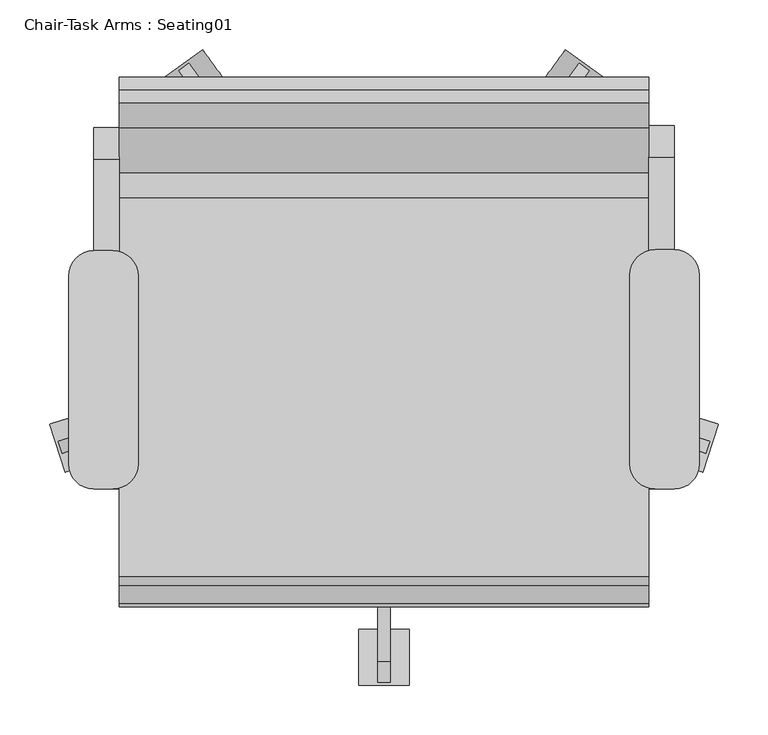
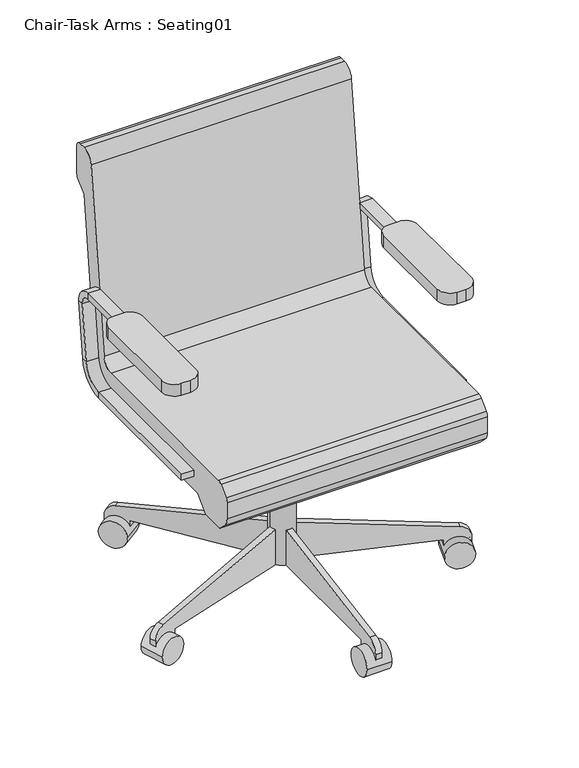
"""IFC4 building model written with IfcOpenShell, lengths in millimetres: furniture geometry, Chair-Task Arms : Seating01."""

from ifc_helpers import new_model, si_unit, point, frame, frame_2d, origin, place, context, project, spatial, polyline, circle_curve, trimmed, segment, composite_curve, outline, extrude, source, transform, mapped, element, save
from ifc_brep_helpers import plane_surface, cylinder_surface, revolved_surface, advanced_brep


def chair_task_arms_seating01_8395c10b(model_context):
    return source(origin(), model_context, "Body", "SolidModel", [
        extrude(outline(composite_curve([segment(trimmed(circle_curve(frame_2d((433.0908197, 48.8028048)), 25.4), [point((433.0908197, 74.2028048))], [point((458.4908197, 48.8028048))], False, "CARTESIAN"), True, "CONTINUOUS"), segment(polyline([(458.4908197, 48.8028048), (458.4908197, -141.6319091)]), True, "CONTINUOUS"), segment(trimmed(circle_curve(frame_2d((433.0908197, -141.6319091)), 25.4), [point((458.4908197, -141.6319091))], [point((433.0908197, -167.0319091))], False, "CARTESIAN"), True, "CONTINUOUS"), segment(polyline([(433.0908197, -167.0319091), (414.0408197, -167.0319091)]), True, "CONTINUOUS"), segment(trimmed(circle_curve(frame_2d((414.0408197, -141.6319091)), 25.4), [point((414.0408197, -167.0319091))], [point((388.6408197, -141.6319091))], False, "CARTESIAN"), True, "CONTINUOUS"), segment(polyline([(388.6408197, -141.6319091), (388.6408197, 48.8028048)]), True, "CONTINUOUS"), segment(trimmed(circle_curve(frame_2d((414.0408197, 48.8028048)), 25.4), [point((388.6408197, 48.8028048))], [point((414.0408197, 74.2028048))], False, "CARTESIAN"), True, "CONTINUOUS"), segment(polyline([(414.0408197, 74.2028048), (433.0908197, 74.2028048)]), True, "CONTINUOUS")], self_intersect=False)), frame((0.0, 0.0, 596.9), z_axis=(0.0, 0.0, 1.0), x_axis=(1.0, 0.0, 0.0)), (0.0, 0.0, 1.0), 25.4),
        extrude(outline(composite_curve([segment(trimmed(circle_curve(frame_2d((-132.0591803, 47.7575984)), 25.4), [point((-132.0591803, 73.1575984))], [point((-106.6591803, 47.7575984))], False, "CARTESIAN"), True, "CONTINUOUS"), segment(polyline([(-106.6591803, 47.7575984), (-106.6591803, -141.6319091)]), True, "CONTINUOUS"), segment(trimmed(circle_curve(frame_2d((-132.0591803, -141.6319091)), 25.4), [point((-106.6591803, -141.6319091))], [point((-132.0591803, -167.0319091))], False, "CARTESIAN"), True, "CONTINUOUS"), segment(polyline([(-132.0591803, -167.0319091), (-151.1091803, -167.0319091)]), True, "CONTINUOUS"), segment(trimmed(circle_curve(frame_2d((-151.1091803, -141.6319091)), 25.4), [point((-151.1091803, -167.0319091))], [point((-176.5091803, -141.6319091))], False, "CARTESIAN"), True, "CONTINUOUS"), segment(polyline([(-176.5091803, -141.6319091), (-176.5091803, 47.7575984)]), True, "CONTINUOUS"), segment(trimmed(circle_curve(frame_2d((-151.1091803, 47.7575984)), 25.4), [point((-176.5091803, 47.7575984))], [point((-151.1091803, 73.1575984))], False, "CARTESIAN"), True, "CONTINUOUS"), segment(polyline([(-151.1091803, 73.1575984), (-132.0591803, 73.1575984)]), True, "CONTINUOUS")], self_intersect=False)), frame((0.0, 0.0, 596.9), z_axis=(0.0, 0.0, 1.0), x_axis=(1.0, 0.0, 0.0)), (0.0, 0.0, 1.0), 25.4),
        advanced_brep(
        [(-151.1091803, -167.0319091, 412.75), (-125.7091803, -167.0319091, 412.75), (-125.7091803, -167.0319091, 425.45), (-151.1091803, -167.0319091, 425.45), (-151.1091803, 126.2388651, 425.45), (-151.1091803, 126.2388651, 412.75), (-125.7091803, 126.2388651, 425.45), (-125.7091803, 126.2388651, 412.75), (-151.1091803, 170.3844094, 464.7064065), (-151.1091803, 182.9974221, 463.2225227), (-125.7091803, 170.3844094, 464.7064065), (-125.7091803, 182.9974221, 463.2225227), (-151.1091803, 184.1806174, 581.9741742), (-151.1091803, 196.7936301, 580.4902904), (-125.7091803, 184.1806174, 581.9741742), (-125.7091803, 196.7936301, 580.4902904), (-151.1091803, 165.2610984, 603.25), (-151.1091803, 165.2610984, 615.95), (-125.7091803, 165.2610984, 603.25), (-125.7091803, 165.2610984, 615.95), (-151.1091803, -18.9459016, 615.95), (-151.1091803, -18.9459016, 603.25), (-125.7091803, -18.9459016, 603.25), (-125.7091803, -18.9459016, 615.95)],
        [
            (0, 1),
            (1, 2),
            (2, 3),
            (3, 0),
            (3, 4),
            (4, 5),
            (5, 0),
            (2, 6),
            (6, 4),
            (1, 7),
            (7, 6),
            (5, 7),
            (8, 9),
            (9, 5, circle_curve(frame((-151.1091803, 126.2388651, 469.9), z_axis=(-1.0, 0.0, 0.0), x_axis=(0.0, 0.0, -1.0)), 57.15)),
            (4, 8, circle_curve(frame((-151.1091803, 126.2388651, 469.9), z_axis=(1.0, 0.0, 0.0), x_axis=(0.0, 0.0, -1.0)), 44.45)),
            (10, 8),
            (6, 10, circle_curve(frame((-125.7091803, 126.2388651, 469.9), z_axis=(1.0, 0.0, 0.0), x_axis=(0.0, 0.0, -1.0)), 44.45)),
            (11, 10),
            (7, 11, circle_curve(frame((-125.7091803, 126.2388651, 469.9), z_axis=(1.0, 0.0, 0.0), x_axis=(0.0, 0.0, -1.0)), 57.15)),
            (9, 11),
            (8, 12),
            (12, 13),
            (13, 9),
            (10, 14),
            (14, 12),
            (11, 15),
            (15, 14),
            (13, 15),
            (16, 17),
            (17, 13, circle_curve(frame((-151.1091803, 165.2610984, 584.2), z_axis=(-1.0, 0.0, 0.0), x_axis=(0.0, 0.9931506043228768, -0.11684124756739202)), 31.75)),
            (12, 16, circle_curve(frame((-151.1091803, 165.2610984, 584.2), z_axis=(1.0, 0.0, 0.0), x_axis=(0.0, 0.9931506043228768, -0.11684124756739202)), 19.05)),
            (18, 16),
            (14, 18, circle_curve(frame((-125.7091803, 165.2610984, 584.2), z_axis=(1.0, 0.0, 0.0), x_axis=(0.0, 0.9931506043228768, -0.11684124756739202)), 19.05)),
            (19, 18),
            (15, 19, circle_curve(frame((-125.7091803, 165.2610984, 584.2), z_axis=(1.0, 0.0, 0.0), x_axis=(0.0, 0.9931506043228768, -0.11684124756739202)), 31.75)),
            (17, 19),
            (20, 21),
            (21, 22),
            (22, 23),
            (23, 20),
            (16, 21),
            (20, 17),
            (18, 22),
            (19, 23),
        ],
        [
            plane_surface(frame((-152.608212, -167.0319091, 419.1), z_axis=(0.0, -1.0, 0.0), x_axis=(0.0, 0.0, -1.0))),
            plane_surface(frame((-151.1091803, -167.0319091, 412.75), z_axis=(-1.0, 0.0, 0.0), x_axis=(0.0, 1.0, 0.0))),
            plane_surface(frame((-151.1091803, -167.0319091, 425.45), z_axis=(0.0, 0.0, 1.0), x_axis=(0.0, 1.0, 0.0))),
            plane_surface(frame((-125.7091803, -167.0319091, 425.45), z_axis=(1.0, 0.0, 0.0), x_axis=(0.0, 1.0, 0.0))),
            plane_surface(frame((-125.7091803, -167.0319091, 412.75), z_axis=(0.0, 0.0, -1.0), x_axis=(0.0, 1.0, 0.0))),
            plane_surface(frame((-151.1091803, 126.2388651, 469.9), z_axis=(-1.0, 0.0, 0.0), x_axis=(0.0, 0.0, -1.0))),
            revolved_surface(polyline([(-151.1091803, 126.2388651, 425.45), (-125.7091803, 126.2388651, 425.45)]), (-138.4091803, 126.2388651, 469.9), (-1.0, 0.0, 0.0)),
            plane_surface(frame((-125.7091803, 126.2388651, 469.9), z_axis=(1.0, 0.0, 0.0), x_axis=(0.0, 0.0, -1.0))),
            cylinder_surface(frame((-138.4091803, 126.2388651, 469.9), z_axis=(-1.0, 0.0, 0.0), x_axis=(0.0, 0.0, -1.0)), 57.15),
            plane_surface(frame((-151.1091803, 182.9974221, 463.2225227), z_axis=(-1.0, 0.0, 0.0), x_axis=(0.0, 0.1168412475673856, 0.9931506043228776))),
            plane_surface(frame((-151.1091803, 170.3844094, 464.7064065), z_axis=(0.0, -0.9931506043228776, 0.1168412475673856), x_axis=(0.0, 0.1168412475673856, 0.9931506043228776))),
            plane_surface(frame((-125.7091803, 170.3844094, 464.7064065), z_axis=(1.0, 0.0, 0.0), x_axis=(0.0, 0.1168412475673856, 0.9931506043228776))),
            plane_surface(frame((-125.7091803, 182.9974221, 463.2225227), z_axis=(0.0, 0.9931506043228776, -0.1168412475673856), x_axis=(0.0, 0.1168412475673856, 0.9931506043228776))),
            plane_surface(frame((-151.1091803, 165.2610984, 584.2), z_axis=(-1.0, 0.0, 0.0), x_axis=(0.0, 0.9931506043228768, -0.11684124756739202))),
            revolved_surface(polyline([(-151.1091803, 184.1806174123508, 581.9741742338413), (-125.7091803, 184.1806174123508, 581.9741742338413)]), (-138.4091803, 165.2610984, 584.2), (-1.0, 0.0, 0.0)),
            plane_surface(frame((-125.7091803, 165.2610984, 584.2), z_axis=(1.0, 0.0, 0.0), x_axis=(0.0, 0.9931506043228768, -0.11684124756739202))),
            cylinder_surface(frame((-138.4091803, 165.2610984, 584.2), z_axis=(-1.0, 0.0, 0.0), x_axis=(0.0, 0.9931506043228768, -0.11684124756739202)), 31.75),
            plane_surface(frame((-152.608212, -18.9459016, 609.6), z_axis=(0.0, -1.0, 0.0), x_axis=(0.0, 0.0, 1.0))),
            plane_surface(frame((-151.1091803, 165.2610984, 615.95), z_axis=(-1.0, 0.0, 0.0), x_axis=(0.0, -1.0, 0.0))),
            plane_surface(frame((-151.1091803, 165.2610984, 603.25), z_axis=(0.0, 0.0, -1.0), x_axis=(0.0, -1.0, 0.0))),
            plane_surface(frame((-125.7091803, 165.2610984, 603.25), z_axis=(1.0, 0.0, 0.0), x_axis=(0.0, -1.0, 0.0))),
            plane_surface(frame((-125.7091803, 165.2610984, 615.95), z_axis=(0.0, 0.0, 1.0), x_axis=(0.0, -1.0, 0.0))),
        ],
        [
            (0, [[1, 2, 3, 4]]),
            (1, [[5, 6, 7, -4]]),
            (2, [[8, 9, -5, -3]]),
            (3, [[10, 11, -8, -2]]),
            (4, [[-7, 12, -10, -1]]),
            (5, [[13, 14, -6, 15]]),
            (6, [[16, -15, -9, 17]]),
            (7, [[18, -17, -11, 19]]),
            (8, [[20, -19, -12, -14]]),
            (9, [[21, 22, 23, -13]]),
            (10, [[24, 25, -21, -16]]),
            (11, [[26, 27, -24, -18]]),
            (12, [[-23, 28, -26, -20]]),
            (13, [[29, 30, -22, 31]]),
            (14, [[32, -31, -25, 33]]),
            (15, [[34, -33, -27, 35]]),
            (16, [[36, -35, -28, -30]]),
            (17, [[37, 38, 39, 40]]),
            (18, [[41, -37, 42, -29]]),
            (19, [[43, -38, -41, -32]]),
            (20, [[44, -39, -43, -34]]),
            (21, [[-42, -40, -44, -36]]),
        ],
    ),
        advanced_brep(
        [(433.0908197, -167.0319091, 425.45), (407.6908197, -167.0319091, 425.45), (407.6908197, -167.0319091, 412.75), (433.0908197, -167.0319091, 412.75), (433.0908197, 128.329278, 412.75), (433.0908197, 128.329278, 425.45), (407.6908197, 128.329278, 412.75), (407.6908197, 128.329278, 425.45), (433.0908197, 185.0878351, 463.2225227), (433.0908197, 172.4748224, 464.7064065), (407.6908197, 185.0878351, 463.2225227), (407.6908197, 172.4748224, 464.7064065), (433.0908197, 198.884043, 580.4902904), (433.0908197, 186.2710303, 581.9741742), (407.6908197, 198.884043, 580.4902904), (407.6908197, 186.2710303, 581.9741742), (433.0908197, 167.3515113, 615.95), (433.0908197, 167.3515113, 603.25), (407.6908197, 167.3515113, 615.95), (407.6908197, 167.3515113, 603.25), (433.0908197, -18.9459016, 603.25), (433.0908197, -18.9459016, 615.95), (407.6908197, -18.9459016, 615.95), (407.6908197, -18.9459016, 603.25)],
        [
            (0, 1),
            (1, 2),
            (2, 3),
            (3, 0),
            (3, 4),
            (4, 5),
            (5, 0),
            (2, 6),
            (6, 4),
            (1, 7),
            (7, 6),
            (5, 7),
            (8, 9),
            (9, 5, circle_curve(frame((433.0908197, 128.329278, 469.9), z_axis=(-1.0, 0.0, 0.0), x_axis=(0.0, 0.0, -1.0)), 44.45)),
            (4, 8, circle_curve(frame((433.0908197, 128.329278, 469.9), z_axis=(1.0, 0.0, 0.0), x_axis=(0.0, 0.0, -1.0)), 57.15)),
            (10, 8),
            (6, 10, circle_curve(frame((407.6908197, 128.329278, 469.9), z_axis=(1.0, 0.0, 0.0), x_axis=(0.0, 0.0, -1.0)), 57.15)),
            (11, 10),
            (7, 11, circle_curve(frame((407.6908197, 128.329278, 469.9), z_axis=(1.0, 0.0, 0.0), x_axis=(0.0, 0.0, -1.0)), 44.45)),
            (9, 11),
            (8, 12),
            (12, 13),
            (13, 9),
            (10, 14),
            (14, 12),
            (11, 15),
            (15, 14),
            (13, 15),
            (16, 17),
            (17, 13, circle_curve(frame((433.0908197, 167.3515113, 584.2), z_axis=(-1.0, 0.0, 0.0), x_axis=(0.0, 0.9931506043228767, -0.1168412475673929)), 19.05)),
            (12, 16, circle_curve(frame((433.0908197, 167.3515113, 584.2), z_axis=(1.0, 0.0, 0.0), x_axis=(0.0, 0.9931506043228767, -0.1168412475673929)), 31.75)),
            (18, 16),
            (14, 18, circle_curve(frame((407.6908197, 167.3515113, 584.2), z_axis=(1.0, 0.0, 0.0), x_axis=(0.0, 0.9931506043228767, -0.1168412475673929)), 31.75)),
            (19, 18),
            (15, 19, circle_curve(frame((407.6908197, 167.3515113, 584.2), z_axis=(1.0, 0.0, 0.0), x_axis=(0.0, 0.9931506043228767, -0.1168412475673929)), 19.05)),
            (17, 19),
            (20, 21),
            (21, 22),
            (22, 23),
            (23, 20),
            (16, 21),
            (20, 17),
            (18, 22),
            (19, 23),
        ],
        [
            plane_surface(frame((406.191788, -167.0319091, 419.1), z_axis=(0.0, -1.0, 0.0), x_axis=(0.0, 0.0, -1.0))),
            plane_surface(frame((433.0908197, -167.0319091, 425.45), z_axis=(1.0, 0.0, 0.0), x_axis=(0.0, 1.0, 0.0))),
            plane_surface(frame((433.0908197, -167.0319091, 412.75), z_axis=(0.0, 0.0, -1.0), x_axis=(0.0, 1.0, 0.0))),
            plane_surface(frame((407.6908197, -167.0319091, 412.75), z_axis=(-1.0, 0.0, 0.0), x_axis=(0.0, 1.0, 0.0))),
            plane_surface(frame((407.6908197, -167.0319091, 425.45), z_axis=(0.0, 0.0, 1.0), x_axis=(0.0, 1.0, 0.0))),
            plane_surface(frame((433.0908197, 128.329278, 469.9), z_axis=(1.0, 0.0, 0.0), x_axis=(0.0, 0.0, -1.0))),
            cylinder_surface(frame((420.3908197, 128.329278, 469.9), z_axis=(-1.0, 0.0, 0.0), x_axis=(0.0, 0.0, -1.0)), 57.15),
            plane_surface(frame((407.6908197, 128.329278, 469.9), z_axis=(-1.0, 0.0, 0.0), x_axis=(0.0, 0.0, -1.0))),
            revolved_surface(polyline([(407.6908197, 128.329278, 425.45), (433.0908197, 128.329278, 425.45)]), (420.3908197, 128.329278, 469.9), (-1.0, 0.0, 0.0)),
            plane_surface(frame((433.0908197, 172.4748224, 464.7064065), z_axis=(1.0, 0.0, 0.0), x_axis=(0.0, 0.11684124756738626, 0.9931506043228775))),
            plane_surface(frame((433.0908197, 185.0878351, 463.2225227), z_axis=(0.0, 0.9931506043228775, -0.11684124756738619), x_axis=(0.0, 0.11684124756738619, 0.9931506043228775))),
            plane_surface(frame((407.6908197, 185.0878351, 463.2225227), z_axis=(-1.0, 0.0, 0.0), x_axis=(0.0, 0.11684124756738619, 0.9931506043228775))),
            plane_surface(frame((407.6908197, 172.4748224, 464.7064065), z_axis=(0.0, -0.9931506043228775, 0.11684124756738626), x_axis=(0.0, 0.11684124756738626, 0.9931506043228775))),
            plane_surface(frame((433.0908197, 167.3515113, 584.2), z_axis=(1.0, 0.0, 0.0), x_axis=(0.0, 0.9931506043228767, -0.1168412475673929))),
            cylinder_surface(frame((420.3908197, 167.3515113, 584.2), z_axis=(-1.0, 0.0, 0.0), x_axis=(0.0, 0.9931506043228767, -0.1168412475673929)), 31.75),
            plane_surface(frame((407.6908197, 167.3515113, 584.2), z_axis=(-1.0, 0.0, 0.0), x_axis=(0.0, 0.9931506043228767, -0.1168412475673929))),
            revolved_surface(polyline([(407.6908197, 186.2710303123508, 581.9741742338412), (433.0908197, 186.2710303123508, 581.9741742338412)]), (420.3908197, 167.3515113, 584.2), (-1.0, 0.0, 0.0)),
            plane_surface(frame((406.191788, -18.9459016, 609.6), z_axis=(0.0, -1.0, 0.0), x_axis=(0.0, 0.0, 1.0))),
            plane_surface(frame((433.0908197, 167.3515113, 603.25), z_axis=(1.0, 0.0, 0.0), x_axis=(0.0, -1.0, 0.0))),
            plane_surface(frame((433.0908197, 167.3515113, 615.95), z_axis=(0.0, 0.0, 1.0), x_axis=(0.0, -1.0, 0.0))),
            plane_surface(frame((407.6908197, 167.3515113, 615.95), z_axis=(-1.0, 0.0, 0.0), x_axis=(0.0, -1.0, 0.0))),
            plane_surface(frame((407.6908197, 167.3515113, 603.25), z_axis=(0.0, 0.0, -1.0), x_axis=(0.0, -1.0, 0.0))),
        ],
        [
            (0, [[1, 2, 3, 4]]),
            (1, [[5, 6, 7, -4]]),
            (2, [[8, 9, -5, -3]]),
            (3, [[10, 11, -8, -2]]),
            (4, [[-7, 12, -10, -1]]),
            (5, [[13, 14, -6, 15]]),
            (6, [[16, -15, -9, 17]]),
            (7, [[18, -17, -11, 19]]),
            (8, [[20, -19, -12, -14]]),
            (9, [[21, 22, 23, -13]]),
            (10, [[24, 25, -21, -16]]),
            (11, [[26, 27, -24, -18]]),
            (12, [[-23, 28, -26, -20]]),
            (13, [[29, 30, -22, 31]]),
            (14, [[32, -31, -25, 33]]),
            (15, [[34, -33, -27, 35]]),
            (16, [[36, -35, -28, -30]]),
            (17, [[37, 38, 39, 40]]),
            (18, [[41, -37, 42, -29]]),
            (19, [[43, -38, -41, -32]]),
            (20, [[44, -39, -43, -34]]),
            (21, [[-42, -40, -44, -36]]),
        ],
    ),
        extrude(outline(composite_curve([segment(trimmed(circle_curve(frame_2d((140.9908197, -18.9459016)), 25.4), [point((115.5908197, -18.9459016))], [point((166.3908197, -18.9459016))], False, "CARTESIAN"), True, "CONTINUOUS"), segment(trimmed(circle_curve(frame_2d((140.9908197, -18.9459016)), 25.4), [point((166.3908197, -18.9459016))], [point((115.5908197, -18.9459016))], False, "CARTESIAN"), True, "CONTINUOUS")], self_intersect=False)), frame((0.0, 0.0, 53.5835944), z_axis=(0.0, 0.0, 1.0), x_axis=(1.0, 0.0, 0.0)), (0.0, 0.0, 1.0), 330.5914056),
        extrude(outline(composite_curve([segment(trimmed(circle_curve(frame_2d((0.0, 28.2002728)), 28.2002727), [point((0.0, 56.4005455))], [point((0.0, 0.0))], False, "CARTESIAN"), True, "CONTINUOUS"), segment(trimmed(circle_curve(frame_2d((0.0, 28.2002728)), 28.2002727), [point((0.0, 0.0))], [point((0.0, 56.4005455))], False, "CARTESIAN"), True, "CONTINUOUS")], self_intersect=False)), frame((461.9222851, -149.9299964, 28.1835944), z_axis=(0.3090169943749423, 0.9510565162951553, 0.0), x_axis=(0.0, 0.0, -1.0)), (0.0, 0.0, 1.0), 50.8),
        extrude(outline(composite_curve([segment(polyline([(25.4, 0.0), (0.0, 0.0), (0.0, 50.8), (24.303053, 50.8)]), True, "CONTINUOUS"), segment(trimmed(circle_curve(frame_2d((24.303053, 25.4)), 25.4), [point((24.303053, 50.8))], [point((49.3171699, 29.8106636))], False, "CARTESIAN"), True, "CONTINUOUS"), segment(polyline([(49.3171699, 29.8106636), (101.6, -266.7), (101.6, -292.1), (25.4, -292.1), (25.4, 0.0)]), True, "CONTINUOUS")], self_intersect=False)), frame((416.8321702, -115.2489746, 28.1835944), z_axis=(0.3090169943749423, 0.9510565162951553, 0.0), x_axis=(0.0, 0.0, 1.0)), (0.0, 0.0, 1.0), 12.7),
        extrude(outline(composite_curve([segment(trimmed(circle_curve(frame_2d((0.0, 28.2002726)), 28.2002727), [point((0.0, 56.4005454))], [point((0.0, 0.0))], False, "CARTESIAN"), True, "CONTINUOUS"), segment(trimmed(circle_curve(frame_2d((0.0, 28.2002726)), 28.2002727), [point((0.0, 0.0))], [point((0.0, 56.4005454))], False, "CARTESIAN"), True, "CONTINUOUS")], self_intersect=False)), frame((364.7373733, 245.8017485, 28.1835944), z_axis=(-0.8090169943749499, 0.5877852522924699, 0.0), x_axis=(0.0, 0.0, -1.0)), (0.0, 0.0, 1.0), 50.8),
        extrude(outline(composite_curve([segment(polyline([(25.4, 0.0), (0.0, 0.0), (0.0, 50.8), (24.303053, 50.8)]), True, "CONTINUOUS"), segment(trimmed(circle_curve(frame_2d((24.303053, 25.3999999)), 25.4), [point((24.303053, 50.8))], [point((49.3171699, 29.8106637))], False, "CARTESIAN"), True, "CONTINUOUS"), segment(polyline([(49.3171699, 29.8106637), (101.6, -266.7), (101.6, -292.1), (25.4, -292.1), (25.4, 0.0)]), True, "CONTINUOUS")], self_intersect=False)), frame((317.8201498, 213.6355261, 28.1835944), z_axis=(-0.8090169943749499, 0.5877852522924699, 0.0), x_axis=(0.0, 0.0, 1.0)), (0.0, 0.0, 1.0), 12.7),
        extrude(outline(composite_curve([segment(trimmed(circle_curve(frame_2d((0.0, 28.2002726)), 28.2002727), [point((0.0, 56.4005454))], [point((0.0, 0.0))], False, "CARTESIAN"), True, "CONTINUOUS"), segment(trimmed(circle_curve(frame_2d((0.0, 28.2002726)), 28.2002727), [point((0.0, 0.0))], [point((0.0, 56.4005454))], False, "CARTESIAN"), True, "CONTINUOUS")], self_intersect=False)), frame((-82.755734, 245.8017485, 28.1835944), z_axis=(0.8090169943749458, 0.5877852522924754, 0.0), x_axis=(0.0, 0.0, 1.0)), (0.0, 0.0, 1.0), 50.8),
        extrude(outline(composite_curve([segment(polyline([(-25.4, 0.0), (-25.4, -292.1), (-101.6, -292.1), (-101.6, -266.6999999), (-49.3171699, 29.8106637)]), True, "CONTINUOUS"), segment(trimmed(circle_curve(frame_2d((-24.303053, 25.3999999)), 25.4), [point((-49.3171699, 29.8106637))], [point((-24.303053, 50.8))], False, "CARTESIAN"), True, "CONTINUOUS"), segment(polyline([(-24.303053, 50.8), (0.0, 50.8), (0.0, 0.0), (-25.4, 0.0)]), True, "CONTINUOUS")], self_intersect=False)), frame((-35.8385104, 213.6355261, 28.1835944), z_axis=(0.8090169943749459, 0.5877852522924754, 0.0), x_axis=(0.0, 0.0, -1.0)), (0.0, 0.0, 1.0), 12.7),
        extrude(outline(composite_curve([segment(trimmed(circle_curve(frame_2d((0.0, 28.2002727)), 28.2002727), [point((0.0, 56.4005454))], [point((0.0, 0.0))], False, "CARTESIAN"), True, "CONTINUOUS"), segment(trimmed(circle_curve(frame_2d((0.0, 28.2002727)), 28.2002727), [point((0.0, 0.0))], [point((0.0, 56.4005454))], False, "CARTESIAN"), True, "CONTINUOUS")], self_intersect=False)), frame((-179.9406457, -149.9299964, 28.1835944), z_axis=(-0.3090169943749487, 0.9510565162951532, 0.0), x_axis=(0.0, 0.0, 1.0)), (0.0, 0.0, 1.0), 50.8),
        extrude(outline(composite_curve([segment(polyline([(-25.4, 0.0), (-25.4, -292.1), (-101.6, -292.1), (-101.6, -266.7), (-49.3171699, 29.8106637)]), True, "CONTINUOUS"), segment(trimmed(circle_curve(frame_2d((-24.303053, 25.4)), 25.4), [point((-49.3171699, 29.8106637))], [point((-24.303053, 50.8000001))], False, "CARTESIAN"), True, "CONTINUOUS"), segment(polyline([(-24.303053, 50.8000001), (0.0, 50.8000001), (0.0, 0.0), (-25.4, 0.0)]), True, "CONTINUOUS")], self_intersect=False)), frame((-134.8505308, -115.2489746, 28.1835944), z_axis=(-0.3090169943749487, 0.9510565162951532, 0.0), x_axis=(0.0, 0.0, -1.0)), (0.0, 0.0, 1.0), 12.7),
        extrude(outline(composite_curve([segment(trimmed(circle_curve(frame_2d((-336.4459016, 28.1835944)), 28.2002727), [point((-308.2456289, 28.1835944))], [point((-364.6461744, 28.1835944))], False, "CARTESIAN"), True, "CONTINUOUS"), segment(trimmed(circle_curve(frame_2d((-336.4459016, 28.1835944)), 28.2002727), [point((-364.6461744, 28.1835944))], [point((-308.2456289, 28.1835944))], False, "CARTESIAN"), True, "CONTINUOUS")], self_intersect=False)), frame((115.5908197, 0.0, 0.0), z_axis=(1.0, 0.0, 0.0), x_axis=(0.0, 1.0, 0.0)), (0.0, 0.0, 1.0), 50.8),
        extrude(outline(composite_curve([segment(polyline([(-311.0459016, 53.5835944), (-311.0459016, 28.1835944), (-361.8459016, 28.1835944), (-361.8459016, 52.4866474)]), True, "CONTINUOUS"), segment(trimmed(circle_curve(frame_2d((-336.4459016, 52.4866474)), 25.4), [point((-361.8459016, 52.4866474))], [point((-340.8565654, 77.5007643))], False, "CARTESIAN"), True, "CONTINUOUS"), segment(polyline([(-340.8565654, 77.5007643), (-44.3459016, 129.7835944), (-18.9459016, 129.7835944), (-18.9459016, 53.5835944), (-311.0459016, 53.5835944)]), True, "CONTINUOUS")], self_intersect=False)), frame((134.6408197, 0.0, 0.0), z_axis=(1.0, 0.0, 0.0), x_axis=(0.0, 1.0, 0.0)), (0.0, 0.0, 1.0), 12.7),
        extrude(outline(polyline([(-69.7459016, 383.7835944), (19.1540984, 383.7835944), (19.1540984, 283.0954134), (-18.9459016, 283.0954134), (-69.7459016, 371.0835944), (-69.7459016, 383.7835944)])), frame((90.1908197, 0.0, 0.0), z_axis=(1.0, 0.0, 0.0), x_axis=(0.0, 1.0, 0.0)), (0.0, 0.0, 1.0), 101.6),
        extrude(outline(composite_curve([segment(trimmed(circle_curve(frame_2d((126.2050455, 482.6)), 25.4), [point((126.2050455, 457.2))], [point((151.4310708, 479.6322323))], True, "CARTESIAN"), True, "CONTINUOUS"), segment(polyline([(151.4310708, 479.6322323), (196.9528985, 866.5677677)]), True, "CONTINUOUS"), segment(trimmed(circle_curve(frame_2d((222.1789239, 863.6)), 25.4), [point((196.9528985, 866.5677677))], [point((222.1789239, 889.0))], False, "CARTESIAN"), True, "CONTINUOUS"), segment(polyline([(222.1789239, 889.0), (235.0540984, 889.0)]), True, "CONTINUOUS"), segment(trimmed(circle_curve(frame_2d((235.0540984, 876.3)), 12.7), [point((235.0540984, 889.0))], [point((247.7540984, 876.3))], False, "CARTESIAN"), True, "CONTINUOUS"), segment(polyline([(247.7540984, 876.3), (247.7540984, 818.0605122)]), True, "CONTINUOUS"), segment(trimmed(circle_curve(frame_2d((235.0540984, 818.0605122)), 12.7), [point((247.7540984, 818.0605122))], [point((244.0343545, 809.0802561))], False, "CARTESIAN"), True, "CONTINUOUS"), segment(polyline([(244.0343545, 809.0802561), (222.3540984, 787.4), (182.7870738, 451.0802913)]), True, "CONTINUOUS"), segment(trimmed(circle_curve(frame_2d((107.1089978, 459.9835944)), 76.2), [point((182.7870738, 451.0802913))], [point((107.1089978, 383.7835944))], False, "CARTESIAN"), True, "CONTINUOUS"), segment(polyline([(107.1089978, 383.7835944), (-181.0744602, 383.7835944), (-209.4470284, 355.6), (-260.2470284, 355.6), (-278.2663256, 373.7401184)]), True, "CONTINUOUS"), segment(trimmed(circle_curve(frame_2d((-260.2459016, 391.6405184)), 25.4), [point((-278.2663256, 373.7401184))], [point((-285.6459016, 391.6405184))], False, "CARTESIAN"), True, "CONTINUOUS"), segment(polyline([(-285.6459016, 391.6405184), (-285.6459016, 426.6837879)]), True, "CONTINUOUS"), segment(trimmed(circle_curve(frame_2d((-272.9459016, 426.6837879)), 12.7), [point((-285.6459016, 426.6837879))], [point((-281.8961016, 435.6939999))], False, "CARTESIAN"), True, "CONTINUOUS"), segment(polyline([(-281.8961016, 435.6939999), (-263.9604301, 453.510212)]), True, "CONTINUOUS"), segment(trimmed(circle_curve(frame_2d((-255.0102301, 444.5)), 12.7), [point((-263.9604301, 453.510212))], [point((-255.0102301, 457.2))], False, "CARTESIAN"), True, "CONTINUOUS"), segment(polyline([(-255.0102301, 457.2), (126.2050455, 457.2)]), True, "CONTINUOUS")], self_intersect=False)), frame((-125.7091803, 0.0, 0.0), z_axis=(1.0, 0.0, 0.0), x_axis=(0.0, 1.0, 0.0)), (0.0, 0.0, 1.0), 533.4),
    ])


if __name__ == "__main__":
    model = new_model("IFC4")
    model_context = context("Model", 3, world=origin())
    ifc_project = project(units=[si_unit("LENGTHUNIT", "METRE", prefix="MILLI")], contexts=[model_context])
    site = spatial("IfcSite", under=ifc_project)
    building = spatial("IfcBuilding", under=site)
    placement = place(None, origin())
    chair_task_arms_seating01_shape = chair_task_arms_seating01_8395c10b(model_context)
    element("IfcFurniture", 1, ObjectType="Chair-Task Arms : Seating01", at=placement, inside=building, context=model_context, shape_type="MappedRepresentation", body=[
        mapped(chair_task_arms_seating01_shape, transform((0.0, 0.0, 0.0), x_axis=(1.0, 0.0, 0.0), y_axis=(0.0, 1.0, 0.0), z_axis=(0.0, 0.0, 1.0))),
    ])
    save(model, "model.ifc")

# Revit data of these elements
# Type "Chair-Task Arms : Seating01"
#   Assembly Code = "E2020200"
#   Seat/Back Material = Textile - Slate Blue
#   Caster Material = Plastic - Black
#   Base Material = Plastic - Black
#   Default Elevation = 0
# Element 1 (IfcFurniture, "Chair-Task Arms : Seating01")
#   Materials on its faces: "Plastic - Black", "Textile - Slate Blue"
# Materials
#   "Textile - Slate Blue": class "Unassigned", colour RGB 98 102 118, transparency 0
#   "Plastic - Black": class "Unassigned", colour RGB 0 0 0, transparency 0.7
